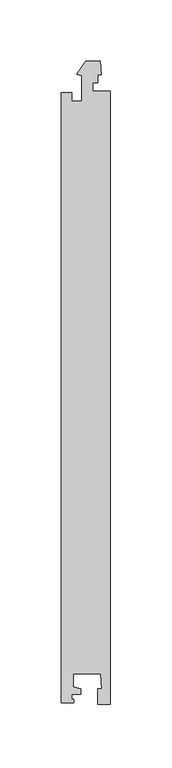
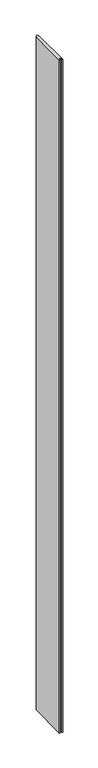
"""IFC4 building model written with IfcOpenShell, lengths in millimetres: proxy geometry, Generic Models 5:Generic Models 5:321804:Generic Models 5:321804 : Generic Models 5:Generic Models 5:321804:33 : Generic Models 5:Generic Models 5:321804:Generic Models 5:321804 : Generic Models 5:Generic Models 5:321804:300761."""

from ifc_helpers import new_model, si_unit, frame, origin, place, context, project, spatial, polyline, outline, extrude, source, transform, mapped, element, save


def generic_models_e18999a9(model_context):
    return source(origin(), model_context, "Body", "SweptSolid", [
        extrude(outline(polyline([(667625.2338797, -492910.833465), (667631.7338797, -492912.5751348), (667631.7338797, -492917.0251348), (667624.2338797, -492917.0251348), (667624.2338797, -492920.9751348), (667625.7338797, -492920.9751348), (667625.7338797, -492923.9751348), (667615.7338797, -492923.9751348), (667615.7338797, -492426.4751348), (667624.2338797, -492426.4751348), (667624.2338797, -492433.4251348), (667632.2338797, -492433.4251348), (667632.2338797, -492412.7091094), (667628.3059983, -492411.6566367), (667635.4133634, -492400.9751348), (667647.2715044, -492400.9751348), (667648.2338797, -492411.9751348), (667645.5338797, -492411.9751348), (667645.5338797, -492418.6001348), (667641.2338797, -492418.6001348), (667641.2338797, -492425.2251348), (667655.7338797, -492425.2251348), (667655.7338797, -492925.2251348), (667645.5338797, -492925.2251348), (667645.5338797, -492912.4751348), (667648.779534, -492912.4751348), (667647.72967, -492900.4751348), (667625.2338797, -492900.4751348), (667625.2338797, -492910.833465)])), frame((0.0, 0.0, -5.8417589), z_axis=(0.0, 0.0, 1.0), x_axis=(1.0, 0.0, 0.0)), (0.0, 0.0, 1.0), 8779.7126309),
    ])


if __name__ == "__main__":
    model = new_model("IFC4")
    model_context = context("Model", 3, world=origin())
    ifc_project = project(units=[si_unit("LENGTHUNIT", "METRE", prefix="MILLI")], contexts=[model_context])
    site = spatial("IfcSite", under=ifc_project)
    building = spatial("IfcBuilding", under=site)
    placement = place(None, origin())
    generic_models_shape = generic_models_e18999a9(model_context)
    element("IfcBuildingElementProxy", 1, Name="Generic Models 5:Generic Models 5:321804:Generic Models 5:321804 : Generic Models 5:Generic Models 5:321804:33 : Generic Models 5:Generic Models 5:321804:Generic Models 5:321804 : Generic Models 5:Generic Models 5:321804:300761", ObjectType="Generic Models 5:Generic Models 5:321804:Generic Models 5:321804 : Generic Models 5:Generic Models 5:321804:33 : Generic Models 5:Generic Models 5:321804:Generic Models 5:321804 : Generic Models 5:Generic Models 5:321804:300761", at=placement, inside=building, context=model_context, shape_type="MappedRepresentation", body=[
        mapped(generic_models_shape, transform((0.0, 0.0, 0.0), x_axis=(1.0, 0.0, 0.0), y_axis=(0.0, 1.0, 0.0), z_axis=(0.0, 0.0, 1.0))),
    ])
    save(model, "model.ifc")

# Revit data of these elements
# Type "Generic Models 5:Generic Models 5:321804:Generic Models 5:321804 : Generic Models 5:Generic Models 5:321804:33 : Generic Models 5:Generic Models 5:321804:Generic Models 5:321804 : Generic Models 5:Generic Models 5:321804:300761"
#   NameOverride = "Generic Models 5:Generic Models 5:321804:Generic Models 5:321804 : Generic Models 5:Generic Models 5:321804:300761"
#   ObjectTypeOverride = "Generic Models 5:321804 : Generic Models 5:Generic Models 5:321804"
#   Reference = "Generic Models 5"
#   Tag = "300761"
# Element 1 (IfcBuildingElementProxy, "Generic Models 5:Generic Models 5:321804:Generic Models 5:321804 : Generic Models 5:Generic Models 5:321804:33 : Generic Models 5:Generic Models 5:321804:Generic Models 5:321804 : Generic Models 5:Generic Models 5:321804:300761")
#   Materials on its faces: "POLYCARBONATE PANEL - ARCOPLUS 547"
# Materials
#   "POLYCARBONATE PANEL - ARCOPLUS 547": class "Unassigned", colour RGB 202 225 249, transparency 0.45, Cost = 0
